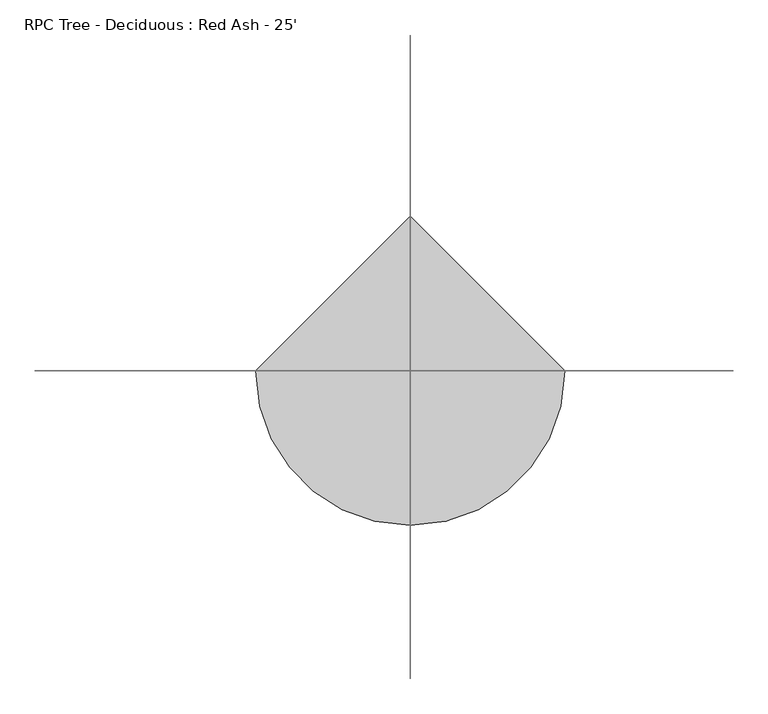
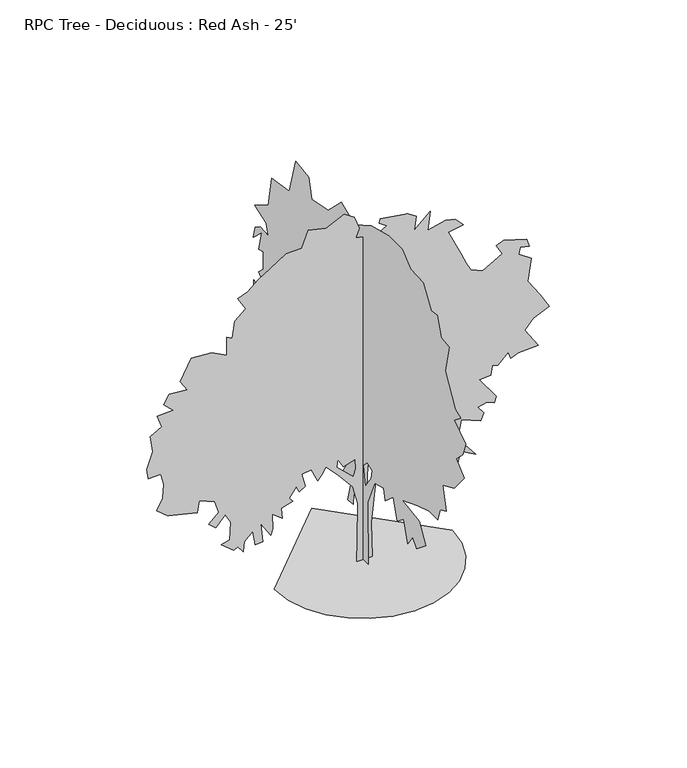
"""IFC4 building model written with IfcOpenShell, lengths in millimetres: geographic element geometry, RPC Tree - Deciduous : Red Ash - 25'."""

from ifc_helpers import new_model, si_unit, origin, place, context, project, spatial, triangles, source, transform, mapped, element, save


def rpc_tree_deciduous_red_ash_25_ab5b1d1a(model_context):
    return source(origin(), model_context, "Body", "Tessellation", [
        triangles([(-1827.1669601, 0.0, 0.0001375), (-1778.8607517, -418.6654335, 0.0001375), (-1641.2908058, -803.1424742, 0.0001375), (-1425.4715664, -1142.4173321, 0.0001375), (-1142.4173321, -1425.4715664, 0.0001375), (-803.1424742, -1641.2908058, 0.0001375), (-418.6648885, -1778.8607517, 0.0001375), (7.99e-05, -1827.1669601, 0.0001375), (418.6654335, -1778.8607517, 0.0001375), (803.1424742, -1641.2908058, 0.0001375), (1142.4173321, -1425.4715664, 0.0001375), (1425.4715664, -1142.4173321, 0.0001375), (1641.2908058, -803.1424742, 0.0001375), (1778.8607517, -418.6648885, 0.0001375), (1827.1669601, 0.0001597, 0.0001375), (-0.0002396, 1827.1669601, 0.0001375), (-0.0001074, -175.219065, 0.0001092), (-6.71e-05, -165.3552049, 1338.5284721), (-6.14e-05, -411.9610099, 1900.7864491), (-7.28e-05, -727.617869, 1989.5653324), (-8.25e-05, -786.7998671, 1752.825713), (-8.8e-05, -1072.8675076, 1999.430864), (-0.0001071, -1210.9627121, 1565.40256), (-0.0001119, -1437.8424683, 1742.9600361), (-0.0001313, -1575.9434864, 1299.0718689), (-0.0001321, -1763.3609711, 1555.5426968), (-0.0001431, -1891.5963123, 1377.9850754), (-0.0001499, -2226.9803467, 1654.1812981), (-0.0001278, -1990.2407272, 2038.8874672), (-9.83e-05, -1388.5203335, 2127.6663506), (-0.0001163, -1931.0529156, 2334.8148983), (-0.0001307, -2345.3501564, 2472.9159164), (-0.0001444, -2651.143119, 2472.9159164), (-0.0001403, -2730.0563255, 2729.386599), (-0.0001471, -2947.0706955, 2828.0253456), (-0.0001271, -2828.7008858, 3321.2414612), (-0.0001396, -3233.1323044, 3508.6590912), (-0.0001428, -3588.2475471, 3932.8218636), (-0.0001224, -3302.1801247, 4189.2925461), (-0.000126, -3529.0598808, 4406.306916), (-0.0001221, -3637.5640137, 4702.2342018), (-9.56e-05, -3223.2669182, 4968.5647476), (-0.0001008, -3469.8719238, 5165.8480545), (-8.99e-05, -3272.5889076, 5234.9013977), (-5.5e-05, -2907.6140923, 5856.3762543), (-4.4e-05, -3055.5748283, 6448.1959442), (-3.03e-05, -2769.5129288, 6477.8104156), (-1.21e-05, -2631.412056, 6882.2479385), (-3.3e-06, -2414.4034996, 6852.6334671), (2.2e-05, -2138.2016087, 7286.6848801), (4.29e-05, -1684.4477646, 7306.3703064), (6.39e-05, -1378.6546566, 7552.980835), (8.53e-05, -905.1696768, 7562.8523254), (0.0001084, -283.725596, 7405.0259125), (0.0001246, 308.1286486, 7059.7591965), (0.0001515, 771.7503496, 7266.9424805), (0.0001587, 1235.3639843, 6813.2056412), (0.0001815, 1817.3589832, 6704.6785446), (0.0001984, 1925.8632614, 7109.1160675), (0.0002211, 2389.482637, 7178.1577835), (0.0002078, 2616.3623932, 6389.0257187), (0.0002331, 3247.668045, 6290.3695313), (0.0002191, 3375.9035316, 5629.4674301), (0.0002313, 3839.5229073, 5343.4052399), (0.0002092, 3444.9568748, 5195.4445038), (0.000199, 3366.0436684, 4968.5647476), (0.0002126, 3652.1055679, 4998.1617783), (0.0002167, 3829.663044, 4869.9262917), (0.0002122, 3898.7108643, 4613.4553185), (0.000207, 3592.9176109, 4899.517218), (0.0001994, 3711.2874207, 4465.4887688), (0.0001934, 3543.5956215, 4514.8110489), (0.0001823, 3553.4610077, 4130.1048798), (0.000185, 3711.2874207, 3982.1441437), (0.0001669, 3464.682415, 3745.3987106), (0.0001678, 3602.7832878, 3567.8467575), (0.0001847, 3888.8451874, 3705.9421074), (0.0001771, 3908.5762505, 3419.8802078), (0.0001628, 3740.8844513, 3193.0062653), (0.00017, 3928.3017906, 3153.549662), (0.0001653, 3967.7583939, 2936.5352921), (0.0001588, 3750.7498375, 3045.0394249), (0.0001388, 3316.7213882, 3025.3141754), (0.0001416, 3701.4278481, 2541.963446), (0.0001321, 3454.8225517, 2591.2857262), (0.000136, 3661.9712448, 2413.7281048), (0.000136, 3859.254261, 2117.8006737), (0.000131, 3721.1530975, 2157.2572769), (0.0001161, 3583.0580383, 1861.3298458), (0.0001212, 3573.1923615, 2048.7531441), (0.0001109, 3296.9903252, 2117.8006737), (0.0001028, 3188.4861923, 2009.2965408), (0.0001016, 2912.2899696, 2384.1371784), (8.9e-05, 2872.8275528, 2019.1620724), (8.43e-05, 2715.0011398, 2098.0752789), (8.28e-05, 2537.4433731, 2315.0895035), (6.8e-05, 2271.1128273, 2216.4450886), (5.8e-05, 2172.4684124, 2029.0219357), (4.86e-05, 2192.1996208, 1683.778038), (3.64e-05, 1985.0510731, 1585.1336231), (3.64e-05, 2083.6896744, 1437.1670734), (3.12e-05, 2133.0118092, 1190.5618498), (1.73e-05, 1689.123642, 1387.8506069), (1.43e-05, 1491.8348122, 1585.1336231), (5.1e-06, 1383.3306793, 1437.1670734), (1.2e-05, 1314.2830044, 1772.5511078), (2.1e-06, 1186.0475904, 1634.4559032), (-1.5e-06, 1038.0810408, 1733.0945045), (2.6e-06, 1057.8121765, 1841.604451), (-4.5e-06, 899.9857635, 1841.604451), (-1.65e-05, 761.8848181, 1644.3214348), (-1.36e-05, 663.2404032, 1890.9267311), (-2.27e-05, 584.3271967, 1703.5034328), (-2.33e-05, 722.4282148, 1476.6294903), (-3.9e-05, 278.5364868, 1614.7246948), (-3.96e-05, 436.3640625, 1358.253867), (-4.61e-05, 554.7344536, 963.6878345), (-5.43e-05, 357.4502747, 983.413302), (-4.92e-05, 327.8575315, 1200.427454), (-5.15e-05, 209.4865591, 1299.0718689), (-5.64e-05, 100.9800372, 1299.0718689), (-6.92e-05, 91.1156048, 884.7746281), (-9.33e-05, 140.4372218, 0.0001186), (-5.08e-05, -313.3189204, 2107.9351421), (-5.47e-05, -283.7261773, 1930.3833344), (-5.43e-05, -76.5775569, 1634.4559032), (-3.89e-05, -7.5275236, 2048.7531441), (-4.09e-05, -145.6269032, 2186.8541622), (133.4683794, 6.11e-05, 2092.498875), (88.4682283, 6.89e-05, 1995.0032272), (73.4677903, 9.59e-05, 1552.5004406), (103.4680849, 0.0001022, 1424.9981941), (178.4673769, 8.15e-05, 1717.502433), (238.4679842, 6.19e-05, 2002.5020428), (-129.0320405, 0.0001973, 0.0), (-121.5315353, 0.0001693, 465.0002506), (-114.0316025, 0.0001215, 1260.0020153), (-211.5318376, 0.0001026, 1650.001902), (-511.5325121, 9.47e-05, 2002.5020428), (-766.5318455, 8.93e-05, 2280.002837), (-826.5335609, 9.9e-05, 2159.9994061), (-931.5337652, 0.0001112, 2032.5028278), (-1059.0302708, 9.98e-05, 2317.5025829), (-1254.0330482, 0.0001101, 2287.5016525), (-1186.5325172, 0.0001242, 2002.5020428), (-1306.5302799, 0.0001339, 1927.5026962), (-1374.0308109, 0.0001288, 2062.4979446), (-1516.5305431, 0.0001471, 1860.0021652), (-1441.5313419, 0.0001492, 1769.9995193), (-1681.5325356, 0.0001637, 1702.4989883), (-1659.0304207, 0.0001766, 1470.0024239), (-1861.5320137, 0.000176, 1627.4997871), (-1854.0331982, 0.000194, 1319.9980625), (-1891.5327988, 0.0002033, 1192.5014843), (-2101.5332073, 0.0001937, 1507.5020245), (-2056.5347912, 0.0002154, 1109.997654), (-2206.5333389, 0.0002228, 1095.0000956), (-2266.5350544, 0.0002071, 1402.5018929), (-2431.5312332, 0.0002242, 1237.4999004), (-2454.0333481, 0.0002377, 1027.4996372), (-2566.5322952, 0.0002337, 1177.498185), (-2649.0359802, 0.0002404, 1125.001026), (-2911.5336205, 0.0002389, 1342.5001774), (-2731.5341423, 0.0002284, 1387.4985935), (-2716.5309883, 0.0002058, 1755.0020336), (-2821.5309746, 0.0001983, 1957.497813), (-3016.5338974, 0.0002194, 1747.5032181), (-3159.0336296, 0.0002184, 1867.5009808), (-2956.5320366, 0.000198, 2062.4979446), (-3039.0301987, 0.0001864, 2317.5025829), (-3361.5352226, 0.0001929, 2444.9990158), (-3399.0349686, 0.0002088, 2205.0036358), (-3999.0349731, 0.0002265, 2347.503368), (-4224.0328674, 0.0002252, 2535.0016617), (-4104.0352501, 0.0002061, 2767.4982262), (-4089.0318054, 0.0001876, 3067.5011353), (-4149.0336662, 0.0001763, 3299.9979904), (-4404.0323456, 0.0001879, 3292.4990295), (-4434.0331306, 0.0001767, 3502.4995834), (-4306.5310295, 0.0001506, 3847.5009087), (-4359.0339294, 0.0001327, 4185.0035637), (-4126.5315514, 0.0001145, 4319.9988121), (-4216.5341972, 0.0001028, 4582.5019753), (-3894.0346962, 8.78e-05, 4597.4996063), (-4089.0318054, 8.52e-05, 4785.0035683), (-3969.0341881, 6.92e-05, 4965.0033371), (-3601.530748, 5.45e-05, 4942.5012222), (-3751.534964, 4.76e-05, 5167.4991165), (-3519.0325859, 1.24e-05, 5587.4996429), (-3106.5307297, -4.3e-06, 5565.0033417), (-2791.5301895, -8.2e-06, 5400.0012039), (-2791.5301895, -3.14e-05, 5789.9896088), (-2679.0312424, -3.28e-05, 5729.9996658), (-2634.0328262, -5.58e-05, 6082.4938477), (-2401.5303028, -7.71e-05, 6269.9922867), (-2574.0309654, -8.61e-05, 6547.4869766), (-2364.0307022, -0.0001002, 6629.9796158), (-2139.0328079, -0.0001212, 6817.4774734), (-1899.0316143, -0.0001406, 6967.5107574), (-1576.5322586, -0.0001672, 7177.5229385), (-1261.5318638, -0.0001815, 7185.0271317), (-1126.5308018, -0.0002075, 7522.5013), (-759.0330299, -0.0002186, 7440.0086609), (-391.5307162, -0.0002454, 7620.0023254), (-181.5309799, -0.0002461, 7477.4738159), (-84.031308, -0.0002338, 7199.9785446), (-151.5312485, -0.0002206, 7027.4896545), (260.9689181, -0.0002328, 6929.9880478), (485.9691015, -0.0002502, 7057.5075897), (328.4688678, -0.0002501, 7170.0181641), (350.9692386, -0.0002564, 7260.0149963), (913.4709143, -0.0002756, 7170.0181641), (1085.9715769, -0.000276, 7050.0033966), (1048.4719036, -0.0002574, 6765.0033508), (1378.4699295, -0.0002897, 7065.0123642), (1318.468214, -0.0002634, 6667.5023254), (1693.4704697, -0.0002851, 6757.4991577), (1880.9687634, -0.0002907, 6712.5292282), (2045.9706104, -0.0002871, 6532.478009), (1745.9677013, -0.0002705, 6472.4991119), (1993.4677105, -0.0002491, 5932.5181183), (2113.4711414, -0.0002391, 5677.5022888), (2203.4679737, -0.0002328, 5505.0017715), (2450.9681282, -0.0002369, 5392.5028244), (2848.4723534, -0.0002681, 5624.9990982), (2720.9699615, -0.0002755, 5842.521286), (2878.4673248, -0.0002864, 5910.0043762), (3350.9710419, -0.0002981, 5760.0001602), (3403.4684189, -0.0002906, 5595.0038361), (3215.9699799, -0.0002846, 5632.5038727), (3185.9691948, -0.0002753, 5497.5028107), (3440.9678741, -0.0002757, 5317.5033325), (3365.9686729, -0.0002443, 4844.9996155), (3620.9673523, -0.0002335, 4477.501989), (3815.9702751, -0.0002224, 4147.5038177), (3478.4676201, -0.0001991, 4004.9982719), (3313.4715866, -0.0001798, 3802.5024925), (3583.467897, -0.000167, 3390.0006363), (3178.4705246, -0.000148, 3367.4985214), (3020.9673477, -0.0001371, 3299.9979904), (2975.9689316, -0.0001436, 3442.5035362), (2758.4697075, -0.0001225, 3247.5006134), (2638.4720901, -0.000119, 3277.5016891), (2615.9699753, -0.000106, 3075.0000961), (2375.9687817, -9.5e-05, 3067.5011353), (2720.9699615, -8.15e-05, 2587.498748), (2683.4705063, -7.18e-05, 2452.5034996), (2533.4718132, -6.93e-05, 2519.998217), (2345.9678513, -5.84e-05, 2474.9998009), (2465.9712822, -5.43e-05, 2317.5025829), (2405.9695667, -4.23e-05, 2159.9994061), (2008.4710098, -3.47e-05, 2325.0012531), (1940.9704788, -8.5e-06, 1935.0015118), (2300.9694351, 3e-06, 1477.5010941), (1993.4677105, 6.2e-06, 1650.001902), (1888.4675789, 3.71e-05, 1207.4990427), (1820.9670479, 2.35e-05, 1484.9999096), (1693.4704697, 1.97e-05, 1642.5030865), (1460.9680916, 3.62e-05, 1537.5029549), (1333.4715134, 5.6e-05, 1297.5016159), (1108.4678782, 4.89e-05, 1582.501371), (890.9687994, 4.01e-05, 1890.0030956), (793.4674107, 5.64e-05, 1687.5015026), (718.4680641, 4e-05, 2017.4995285), (425.9690938, 6.13e-05, 1874.9997963), (260.9689181, 8.46e-05, 1604.9976723), (163.4686739, 0.0001398, 749.9987703), (185.9684634, 0.0001835, 0.0002425), (-406.5323078, 8.11e-05, 2152.5005905), (-519.0324177, 7.4e-05, 2355.0021835), (-541.5322071, 8.48e-05, 2190.0001911), (-204.0319139, 8.97e-05, 1860.0021652), (-151.5318299, 7.8e-05, 2017.4995285), (-166.5316956, 6.62e-05, 2227.4999371)], [[15, 16, 1], [14, 15, 1], [14, 1, 2], [13, 14, 2], [13, 2, 3], [13, 3, 4], [12, 13, 4], [11, 12, 4], [11, 4, 5], [11, 5, 6], [11, 6, 7], [11, 7, 8], [11, 8, 9], [11, 9, 10], [126, 17, 18], [88, 89, 90], [68, 69, 70], [67, 68, 70], [83, 84, 85], [86, 87, 88], [126, 18, 19], [125, 126, 19], [113, 114, 115], [104, 105, 106], [63, 64, 65], [80, 81, 82], [79, 80, 82], [66, 67, 70], [24, 25, 26], [101, 102, 103], [110, 111, 112], [42, 43, 44], [70, 71, 72], [20, 21, 22], [100, 101, 103], [116, 117, 118], [116, 118, 119], [76, 77, 78], [22, 23, 24], [93, 94, 95], [93, 95, 96], [76, 78, 79], [91, 92, 93], [45, 46, 47], [116, 119, 120], [115, 116, 120], [26, 27, 28], [26, 28, 29], [26, 29, 30], [24, 26, 30], [22, 24, 30], [123, 17, 126], [122, 123, 126], [121, 122, 126], [73, 74, 75], [79, 82, 83], [76, 79, 83], [37, 38, 39], [124, 125, 19], [59, 60, 61], [58, 59, 61], [106, 107, 108], [106, 108, 109], [66, 70, 72], [124, 19, 20], [34, 35, 36], [47, 48, 49], [100, 103, 104], [115, 120, 121], [115, 121, 126], [115, 126, 127], [40, 41, 42], [39, 40, 42], [32, 33, 34], [113, 115, 127], [112, 113, 127], [61, 62, 63], [55, 56, 57], [98, 99, 100], [98, 100, 104], [98, 104, 106], [86, 88, 90], [86, 90, 91], [85, 86, 91], [85, 91, 93], [83, 85, 93], [75, 76, 83], [36, 37, 39], [49, 50, 51], [83, 93, 96], [32, 34, 36], [97, 98, 106], [31, 32, 36], [42, 44, 45], [97, 106, 109], [51, 52, 53], [75, 83, 96], [75, 96, 97], [61, 63, 65], [61, 65, 66], [58, 61, 66], [57, 58, 66], [75, 97, 109], [73, 75, 109], [72, 73, 109], [66, 72, 109], [57, 66, 109], [57, 109, 110], [57, 110, 112], [57, 112, 127], [57, 127, 128], [55, 57, 128], [54, 55, 128], [53, 54, 128], [51, 53, 128], [49, 51, 128], [47, 49, 128], [45, 47, 128], [42, 45, 128], [39, 42, 128], [36, 39, 128], [31, 36, 128], [30, 31, 128], [30, 128, 124], [30, 124, 20], [30, 20, 22], [135, 130, 131], [130, 135, 136], [130, 136, 137], [135, 131, 132], [253, 254, 255], [255, 256, 257], [130, 137, 138], [272, 129, 130], [272, 130, 138], [129, 272, 273], [262, 263, 264], [214, 215, 216], [272, 138, 139], [271, 272, 139], [271, 139, 140], [159, 160, 161], [150, 151, 152], [153, 154, 155], [152, 153, 155], [162, 163, 164], [218, 219, 220], [237, 238, 239], [228, 229, 230], [227, 228, 230], [191, 192, 193], [141, 142, 143], [148, 149, 150], [259, 260, 261], [182, 183, 184], [217, 218, 220], [161, 162, 164], [270, 271, 140], [129, 273, 274], [195, 196, 197], [268, 135, 132], [267, 268, 132], [266, 267, 132], [266, 132, 133], [265, 266, 133], [265, 133, 134], [246, 247, 248], [245, 246, 248], [234, 235, 236], [140, 141, 143], [225, 226, 227], [225, 227, 230], [225, 230, 231], [167, 168, 169], [166, 167, 169], [239, 240, 241], [145, 146, 147], [144, 145, 147], [255, 257, 258], [253, 255, 258], [171, 172, 173], [237, 239, 241], [216, 217, 220], [245, 248, 249], [250, 251, 252], [249, 250, 252], [155, 156, 157], [155, 157, 158], [210, 211, 212], [209, 210, 212], [177, 178, 179], [243, 244, 245], [201, 202, 203], [184, 185, 186], [184, 186, 187], [274, 269, 270], [173, 174, 175], [171, 173, 175], [159, 161, 164], [177, 179, 180], [158, 159, 164], [158, 164, 165], [155, 158, 165], [171, 175, 176], [180, 181, 182], [188, 189, 190], [187, 188, 190], [187, 190, 191], [231, 232, 233], [245, 249, 252], [212, 213, 214], [209, 212, 214], [203, 204, 205], [203, 205, 206], [203, 206, 207], [201, 203, 207], [264, 265, 134], [208, 209, 214], [241, 242, 243], [225, 231, 233], [224, 225, 233], [233, 234, 236], [224, 233, 236], [224, 236, 237], [224, 237, 241], [224, 241, 243], [223, 224, 243], [223, 243, 245], [152, 155, 165], [152, 165, 166], [259, 261, 262], [258, 259, 262], [253, 258, 262], [252, 253, 262], [252, 262, 264], [245, 252, 264], [223, 245, 264], [223, 264, 134], [223, 134, 129], [223, 129, 274], [223, 274, 270], [222, 223, 270], [221, 222, 270], [220, 221, 270], [216, 220, 270], [214, 216, 270], [208, 214, 270], [207, 208, 270], [201, 207, 270], [200, 201, 270], [199, 200, 270], [198, 199, 270], [197, 198, 270], [195, 197, 270], [194, 195, 270], [193, 194, 270], [191, 193, 270], [191, 270, 140], [191, 140, 143], [191, 143, 144], [187, 191, 144], [184, 187, 144], [182, 184, 144], [180, 182, 144], [177, 180, 144], [176, 177, 144], [171, 176, 144], [170, 171, 144], [170, 144, 147], [169, 170, 147], [166, 169, 147], [152, 166, 147], [152, 147, 148], [152, 148, 150]], closed=False),
    ])


if __name__ == "__main__":
    model = new_model("IFC4")
    model_context = context("Model", 3, world=origin())
    ifc_project = project(units=[si_unit("LENGTHUNIT", "METRE", prefix="MILLI")], contexts=[model_context])
    site = spatial("IfcSite", under=ifc_project)
    building = spatial("IfcBuilding", under=site)
    placement = place(None, origin())
    rpc_tree_deciduous_red_ash_25_shape = rpc_tree_deciduous_red_ash_25_ab5b1d1a(model_context)
    element("IfcGeographicElement", 1, ObjectType="RPC Tree - Deciduous : Red Ash - 25'", at=placement, inside=building, context=model_context, shape_type="MappedRepresentation", body=[
        mapped(rpc_tree_deciduous_red_ash_25_shape, transform((0.0, 0.0, 0.0), x_axis=(1.0, 0.0, 0.0), y_axis=(0.0, 1.0, 0.0), z_axis=(0.0, 0.0, 1.0))),
    ])
    save(model, "model.ifc")

# Revit data of these elements
# Type "RPC Tree - Deciduous : Red Ash - 25'"
#   built-in parameter 1005195 = "RPC-16-FVGW-4XXX-7J75-W000-ST1L-LVER-AU"
#   Type Comments = "Red Maple"
#   Assembly Code = "G2050500"
#   Height = 7.62 m
#   Default Elevation = 0
